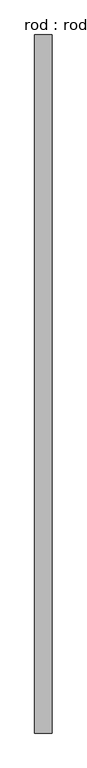
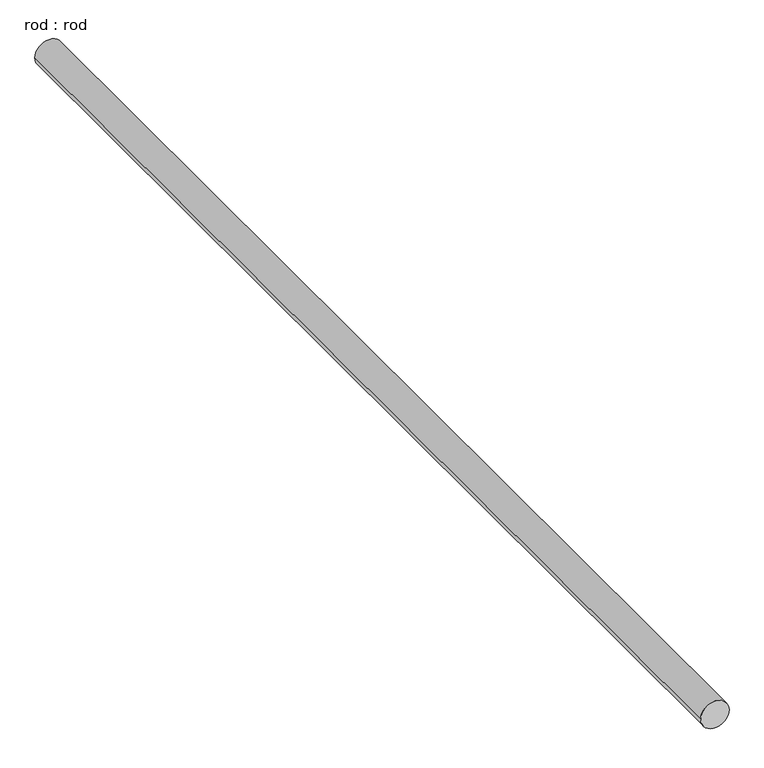
"""IFC4 building model written with IfcOpenShell, lengths in millimetres: proxy geometry, rod : rod."""

from ifc_helpers import new_model, si_unit, point, frame, frame_2d, origin, place, context, project, spatial, circle_curve, trimmed, segment, composite_curve, outline, extrude, source, transform, mapped, element, save


def rod_rod_26737320(model_context):
    return source(origin(), model_context, "Body", "SweptSolid", [
        extrude(outline(composite_curve([segment(trimmed(circle_curve(frame_2d((0.0108462, 0.0)), 200.0), [point((0.0108462, 200.0))], [point((0.0108462, -200.0))], False, "CARTESIAN"), True, "CONTINUOUS"), segment(trimmed(circle_curve(frame_2d((0.0108462, 0.0)), 200.0), [point((0.0108462, -200.0))], [point((0.0108462, 200.0))], False, "CARTESIAN"), True, "CONTINUOUS")], self_intersect=False)), frame((0.0, -4016.8255439, 0.0), z_axis=(0.0, 1.0, 0.0), x_axis=(0.0, 0.0, 1.0)), (0.0, 0.0, 1.0), 16219.1083186),
    ])


if __name__ == "__main__":
    model = new_model("IFC4")
    model_context = context("Model", 3, world=origin())
    ifc_project = project(units=[si_unit("LENGTHUNIT", "METRE", prefix="MILLI")], contexts=[model_context])
    site = spatial("IfcSite", under=ifc_project)
    building = spatial("IfcBuilding", under=site)
    placement = place(None, origin())
    rod_rod_shape = rod_rod_26737320(model_context)
    element("IfcBuildingElementProxy", 1, Name="rod : rod", ObjectType="rod : rod", at=placement, inside=building, context=model_context, shape_type="MappedRepresentation", body=[
        mapped(rod_rod_shape, transform((0.0, 0.0, 0.0), x_axis=(1.0, 0.0, 0.0), y_axis=(0.0, 1.0, 0.0), z_axis=(0.0, 0.0, 1.0))),
    ])
    save(model, "model.ifc")

# Revit data of these elements
# Type "rod : rod"
#   Default Elevation = 0
